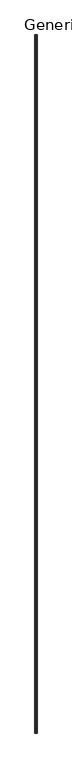
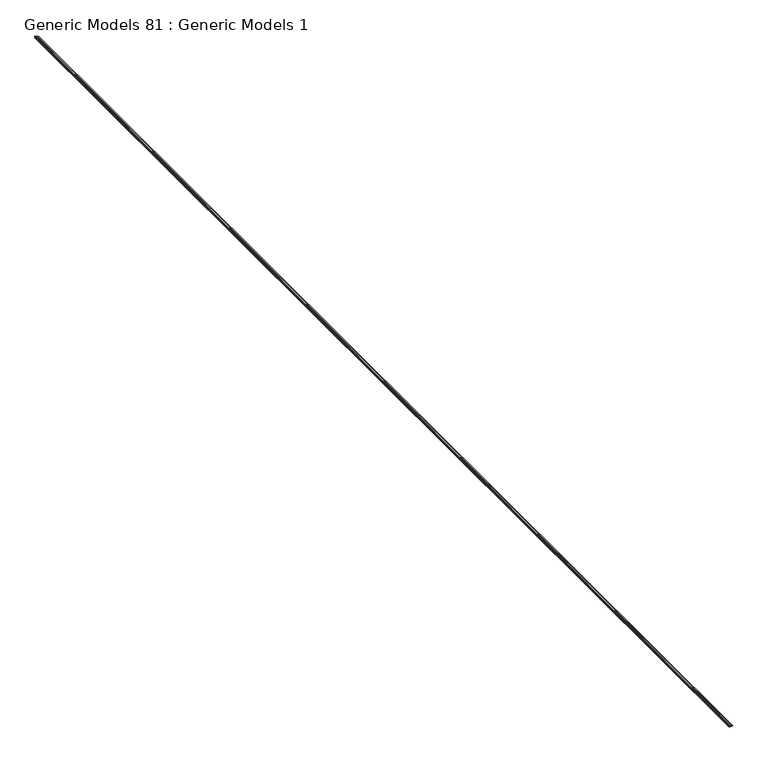
"""IFC4 building model written with IfcOpenShell, lengths in millimetres: proxy geometry, Generic Models 81 : Generic Models 1."""

from ifc_helpers import new_model, si_unit, frame, origin, place, context, project, spatial, polyline, outline, extrude, source, transform, mapped, element, save


def generic_models_81_generic_models_1_07468851(model_context):
    return source(origin(), model_context, "Body", "SweptSolid", [
        extrude(outline(polyline([(142822.070303, -8391.2874704), (142824.280103, -8391.2874704), (142824.280103, -8390.4286296), (142844.5946817, -8390.4286296), (142844.5946817, -8391.6986296), (142825.550103, -8391.6986296), (142825.550103, -8392.5574704), (142820.800303, -8392.5574704), (142820.800303, -8370.3324704), (142832.230303, -8370.3324704), (142832.230303, -8357.6324704), (142820.800303, -8357.6324704), (142820.800303, -8333.9192865), (142822.070303, -8333.9192865), (142822.070303, -8356.3624704), (142833.500303, -8356.3624704), (142833.500303, -8371.6024704), (142822.070303, -8371.6024704), (142822.070303, -8391.2874704)])), frame((0.0, -7068.1230338, 0.0), z_axis=(0.0, 1.0, 0.0), x_axis=(0.0, 0.0, 1.0)), (0.0, 0.0, 1.0), 19050.0),
    ])


if __name__ == "__main__":
    model = new_model("IFC4")
    model_context = context("Model", 3, world=origin())
    ifc_project = project(units=[si_unit("LENGTHUNIT", "METRE", prefix="MILLI")], contexts=[model_context])
    site = spatial("IfcSite", under=ifc_project)
    building = spatial("IfcBuilding", under=site)
    placement = place(None, origin())
    generic_models_81_generic_models_1_shape = generic_models_81_generic_models_1_07468851(model_context)
    element("IfcBuildingElementProxy", 1, Name="Generic Models 81 : Generic Models 1", ObjectType="Generic Models 81 : Generic Models 1", at=placement, inside=building, context=model_context, shape_type="MappedRepresentation", body=[
        mapped(generic_models_81_generic_models_1_shape, transform((0.0, 0.0, 0.0), x_axis=(1.0, 0.0, 0.0), y_axis=(0.0, 1.0, 0.0), z_axis=(0.0, 0.0, 1.0))),
    ])
    save(model, "model.ifc")

# Revit data of these elements
# Element 1 (IfcBuildingElementProxy, "Generic Models 81 : Generic Models 1")
#   Materials on its faces: "_16 GA. COPPER SOFFIT DRIP SCREED"
# Materials
#   "_16 GA. COPPER SOFFIT DRIP SCREED": class "Generic", colour RGB 253 192 103, transparency 0, Cost = 0
